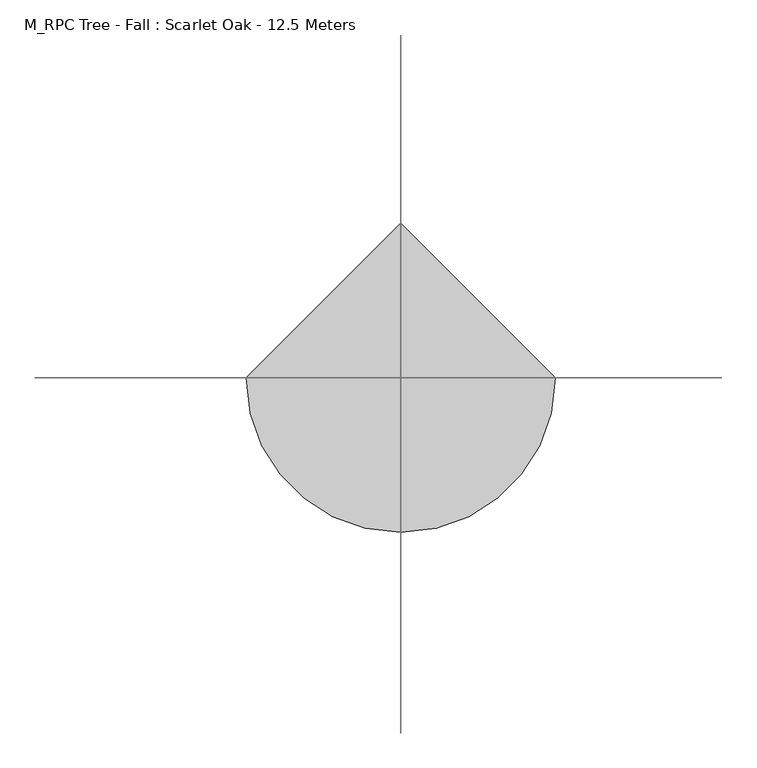
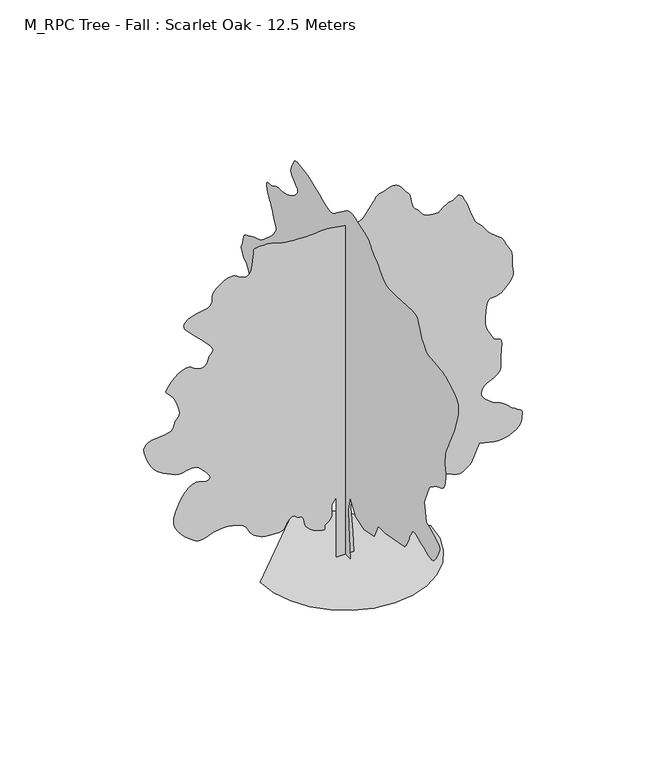
"""IFC4 building model written with IfcOpenShell, lengths in millimetres: geographic element geometry, M_RPC Tree - Fall : Scarlet Oak - 12.5 Meters."""

import ifcopenshell
import ifcopenshell.guid

model = None  # the IFC model being written
_history = None  # IfcOwnerHistory: only IFC2X3 demands one
_inside = {}  # id of a spatial element -> (the spatial element, [elements in it])
_under = {}  # id of a project, library or spatial element -> (it, [spatial elements below it])
_declared = {}  # id of a project -> (the project, [libraries it declares])
_typed = {}  # id of a type object -> (the type object, [elements of that type])
_made_of = {}  # id of a material, layer set ... -> (it, [elements and type objects made of it])


def new_model(schema):
    """Start an empty IFC model of exactly this schema.

    Asked for "IFC4X3", IfcOpenShell would pick the latest addendum, in which some entities
    have other attributes; the version numbers below select the first issue.
    IFC2X3 requires an IfcOwnerHistory on every rooted entity: one is made here for all.
    """
    global model, _history
    if schema == "IFC4X3":
        model = ifcopenshell.file(schema_version=(4, 3, 0, 0))
    else:
        model = ifcopenshell.file(schema=schema)
    _inside.clear()
    _under.clear()
    _declared.clear()
    _typed.clear()
    _made_of.clear()
    _history = None
    if model.schema == "IFC2X3":
        org = make("IfcOrganization", Name="unknown")
        user = make(
            "IfcPersonAndOrganization",
            ThePerson=make("IfcPerson", FamilyName="unknown"),
            TheOrganization=org,
        )
        app = make(
            "IfcApplication",
            ApplicationDeveloper=org,
            Version="unknown",
            ApplicationFullName="unknown",
            ApplicationIdentifier="unknown",
        )
        _history = make(
            "IfcOwnerHistory",
            OwningUser=user,
            OwningApplication=app,
            ChangeAction="ADDED",
            CreationDate=0,
        )
    return model


def make(cls, **values):
    """One entity of the class cls with the attributes given. An attribute that is None is left unset."""
    return model.create_entity(
        cls, **{name: value for name, value in values.items() if value is not None}
    )


def rooted(cls, **values):
    """An entity with a GlobalId (a new one), such as an element, a storey or a relation."""
    return make(cls, GlobalId=ifcopenshell.guid.new(), OwnerHistory=_history, **values)


def si_unit(unit_type, name, prefix=None):
    """IfcSIUnit, for example si_unit("LENGTHUNIT", "METRE", prefix="MILLI")."""
    return make("IfcSIUnit", UnitType=unit_type, Prefix=prefix, Name=name)


def assignment(units):
    """IfcUnitAssignment: the units of a project."""
    return None if units is None else make("IfcUnitAssignment", Units=units)


def point(xyz):
    """IfcCartesianPoint."""
    return None if xyz is None else make("IfcCartesianPoint", Coordinates=xyz)


def direction(xyz):
    """IfcDirection."""
    return None if xyz is None else make("IfcDirection", DirectionRatios=xyz)


def frame(location, z_axis=None, x_axis=None):
    """IfcAxis2Placement3D, a coordinate frame: its origin and axes. An axis left out is left unset."""
    return make(
        "IfcAxis2Placement3D",
        Location=point(location),
        Axis=direction(z_axis),
        RefDirection=direction(x_axis),
    )


def origin():
    """The frame at (0, 0, 0) with its axes left unset."""
    return frame((0.0, 0.0, 0.0))


def place(relative_to, where):
    """IfcLocalPlacement: puts the frame where relative to a parent placement (None: the world)."""
    return make(
        "IfcLocalPlacement", PlacementRelTo=relative_to, RelativePlacement=where
    )


def context(
    kind, dimensions, precision=None, world=None, true_north=None, identifier=None
):
    """IfcGeometricRepresentationContext, for example the 3D "Model" context."""
    return make(
        "IfcGeometricRepresentationContext",
        ContextIdentifier=identifier,
        ContextType=kind,
        CoordinateSpaceDimension=dimensions,
        Precision=precision,
        WorldCoordinateSystem=world,
        TrueNorth=true_north,
    )


def project(units=None, contexts=None):
    """IfcProject with its units and contexts."""
    return rooted(
        "IfcProject",
        Name="project",
        RepresentationContexts=contexts,
        UnitsInContext=assignment(units),
    )


def spatial(cls, under=None, at=None, **own):
    """A site, building, storey or space (cls), placed at a placement, below another one or the project."""
    s = rooted(cls, ObjectPlacement=at, **own)
    if under is not None:
        _under.setdefault(under.id(), (under, []))[1].append(s)
    return s


def point_list(points):
    """IfcCartesianPointList2D or 3D."""
    cls = (
        "IfcCartesianPointList2D" if len(points[0]) == 2 else "IfcCartesianPointList3D"
    )
    return make(cls, CoordList=points)


def triangles(points, corners, closed=None, point_numbers=None):
    """IfcTriangulatedFaceSet: each triangle names its three corners, points numbered from 1."""
    return make(
        "IfcTriangulatedFaceSet",
        Coordinates=point_list(points),
        Closed=closed,
        CoordIndex=corners,
        PnIndex=point_numbers,
    )


def shape(context_of_items, identifier, shape_type, items):
    """IfcShapeRepresentation: the items that make up one representation, for example the "Body"."""
    return make(
        "IfcShapeRepresentation",
        ContextOfItems=context_of_items,
        RepresentationIdentifier=identifier,
        RepresentationType=shape_type,
        Items=items,
    )


def source(mapping_origin, context_of_items, identifier, shape_type, items):
    """IfcRepresentationMap: a shape defined once, which mapped items show again and again."""
    return make(
        "IfcRepresentationMap",
        MappingOrigin=mapping_origin,
        MappedRepresentation=shape(context_of_items, identifier, shape_type, items),
    )


def transform(
    local_origin,
    x_axis=None,
    y_axis=None,
    z_axis=None,
    scale=None,
    scale2=None,
    scale3=None,
    uniform=True,
):
    """IfcCartesianTransformationOperator3D, or its non-uniform kind. x_axis, y_axis, z_axis: its Axis1, 2, 3."""
    if uniform:
        return make(
            "IfcCartesianTransformationOperator3D",
            Axis1=direction(x_axis),
            Axis2=direction(y_axis),
            LocalOrigin=point(local_origin),
            Scale=scale,
            Axis3=direction(z_axis),
        )
    return make(
        "IfcCartesianTransformationOperator3DnonUniform",
        Axis1=direction(x_axis),
        Axis2=direction(y_axis),
        LocalOrigin=point(local_origin),
        Scale=scale,
        Axis3=direction(z_axis),
        Scale2=scale2,
        Scale3=scale3,
    )


def mapped(mapping_source, mapping_target):
    """IfcMappedItem: shows the shape of a source again, moved by a transform."""
    return make(
        "IfcMappedItem", MappingSource=mapping_source, MappingTarget=mapping_target
    )


def made_of(thing, what):
    """Note that an element or type object is made of a material, layer set ...; save() writes the relation."""
    if what is not None:
        _made_of.setdefault(what.id(), (what, []))[1].append(thing)
    return thing


def element(
    cls,
    number,
    at=None,
    inside=None,
    cuts=None,
    type_object=None,
    material=None,
    context=None,
    identifier="Body",
    shape_type=None,
    held_by="IfcProductDefinitionShape",
    body=None,
    shapes=None,
    **own,
):
    """One element of the class cls, such as IfcWall. Its Tag is "e" and its number.

    at: its placement. inside: the storey or other place that contains it. cuts: it is an
    opening in that element (IfcRelVoidsElement). A single representation is given by context,
    identifier, shape_type and body (its items); several are given by shapes. held_by: the class
    of the entity that holds the representations. save() writes the other relations.
    """
    e = rooted(cls, Tag="e%d" % number, ObjectPlacement=at, **own)
    if body is not None:
        shapes = [shape(context, identifier, shape_type, body)]
    if shapes is not None:
        e.Representation = make(held_by, Representations=shapes)
    if inside is not None:
        _inside.setdefault(inside.id(), (inside, []))[1].append(e)
    if cuts is not None:
        rooted(
            "IfcRelVoidsElement", RelatingBuildingElement=cuts, RelatedOpeningElement=e
        )
    if type_object is not None:
        _typed.setdefault(type_object.id(), (type_object, []))[1].append(e)
    return made_of(e, material)


def aggregate(whole, parts):
    """IfcRelAggregates: a whole, such as a stair, and the parts it consists of."""
    return rooted("IfcRelAggregates", RelatingObject=whole, RelatedObjects=parts)


def save(model, path):
    """Write the relations noted so far, then the file.

    IfcRelAggregates (storeys below a building ...), IfcRelContainedInSpatialStructure (elements
    in a storey), IfcRelDefinesByType, IfcRelAssociatesMaterial and IfcRelDeclares: one each for
    every whole, place, type object, material and project.
    """
    for whole, parts in _under.values():
        aggregate(whole, parts)
    for where, things in _inside.values():
        rooted(
            "IfcRelContainedInSpatialStructure",
            RelatedElements=things,
            RelatingStructure=where,
        )
    for kind, things in _typed.values():
        rooted("IfcRelDefinesByType", RelatedObjects=things, RelatingType=kind)
    for what, things in _made_of.values():
        rooted("IfcRelAssociatesMaterial", RelatedObjects=things, RelatingMaterial=what)
    for by, libraries in _declared.values():
        rooted("IfcRelDeclares", RelatingContext=by, RelatedDefinitions=libraries)
    model.write(path)


def m_rpc_tree_fall_scarlet_oak_12_5_meters_13b38d7d(model_context):
    return source(origin(), model_context, "Body", "Tessellation", [
        triangles([(0.0172504, 306.0074844, 0.0), (0.0172504, -293.5650026, 0.0), (0.0172504, -196.8600042, 1141.1199549), (0.0172504, -177.5184886, 1682.6674953), (0.0172504, -293.5650026, 2185.5349113), (0.0172504, -603.0224945, 1682.6674953), (0.0172504, -1105.8875124, 1527.9400211), (0.0172504, -1686.1174301, 1663.3275421), (0.0172504, -1918.2099495, 2146.8525341), (0.0172504, -2324.3725124, 2146.8525341), (0.0172504, -3446.1498253, 2359.6049549), (0.0172504, -3487.4249222, 2409.394939), (0.0172504, -3527.7000801, 2459.5225479), (0.0172504, -3565.9250725, 2510.3249702), (0.0172504, -3601.0999603, 2562.1500046), (0.0172504, -3632.2248047, 2615.3249565), (0.0172504, -3658.2749588, 2670.2000954), (0.0172504, -3678.2499023, 2727.0748215), (0.0172504, -3697.649881, 2785.6750237), (0.0172504, -3722.1248405, 2845.2748741), (0.0172504, -3750.8248329, 2905.7249634), (0.0172504, -3782.89991, 2966.8500114), (0.0172504, -3817.5248314, 3028.475029), (0.0172504, -3853.8249413, 3090.4500252), (0.0172504, -3890.9999977, 3152.5750122), (0.0172504, -3908.7000801, 3172.6499496), (0.0172504, -3933.1750397, 3188.8498329), (0.0172504, -3971.1750458, 3197.2499016), (0.0172504, -4029.4749756, 3193.9748108), (0.0172504, -4114.8499969, 3175.1500877), (0.0172504, -4234.0499886, 3136.8498093), (0.0172504, -4393.8498276, 3075.2250824), (0.0172504, -4562.5749939, 3002.6998581), (0.0172504, -4706.2499451, 2937.9750298), (0.0172504, -4828.2750549, 2886.4249786), (0.0172504, -4932.0251175, 2853.4999535), (0.0172504, -5020.8999252, 2844.5999153), (0.0172504, -5098.249855, 2865.1248253), (0.0172504, -5167.4996979, 2920.4999336), (0.0172504, -5237.3750839, 3007.7248421), (0.0172504, -5309.5997452, 3113.9000473), (0.0172504, -5377.0996948, 3229.5499649), (0.0172504, -5432.7497864, 3345.1998825), (0.0172504, -5469.4498718, 3451.3750877), (0.0172504, -5480.1248016, 3538.6249947), (0.0172504, -5457.6250122, 3597.424894), (0.0172504, -5402.6498795, 3641.6998077), (0.0172504, -5323.3000717, 3691.0249947), (0.0172504, -5223.6747574, 3744.5999222), (0.0172504, -5107.774855, 3801.5499344), (0.0172504, -4979.7251129, 3861.0500816), (0.0172504, -4843.5499947, 3922.224836), (0.0172504, -4703.3248329, 3984.2498291), (0.0172504, -4587.2749397, 4641.8498062), (0.0172504, -4877.3749649, 5318.7747665), (0.0172504, -4886.5249878, 5331.7001404), (0.0172504, -4900.7247025, 5347.4747589), (0.0172504, -4925.0999588, 5369.0251877), (0.0172504, -4964.6748688, 5399.20009), (0.0172504, -5024.5497025, 5440.8498734), (0.0172504, -5109.8247299, 5496.8999405), (0.0172504, -5225.5246445, 5570.225116), (0.0172504, -5351.0501221, 5636.6501312), (0.0172504, -5462.3497238, 5680.0498077), (0.0172504, -5559.4501923, 5715.3499786), (0.0172504, -5642.3497833, 5757.424736), (0.0172504, -5711.0246613, 5821.1499161), (0.0172504, -5765.4998245, 5921.4001923), (0.0172504, -5805.7496933, 6073.0746552), (0.0172504, -5829.0500153, 6222.0498642), (0.0172504, -5835.7501877, 6317.5748474), (0.0172504, -5830.6249191, 6379.6001312), (0.0172504, -5818.3750854, 6428.1000778), (0.0172504, -5803.7748138, 6483.0246323), (0.0172504, -5791.5499786, 6564.3249023), (0.0172504, -5786.4247101, 6691.9996674), (0.0172504, -5788.2251816, 6832.849791), (0.0172504, -5796.1246994, 6949.6746368), (0.0172504, -5813.8247818, 7056.3751007), (0.0172504, -5845.0496201, 7166.7747574), (0.0172504, -5893.550148, 7294.7750839), (0.0172504, -5963.0249771, 7454.2496521), (0.0172504, -6057.1750443, 7659.049942), (0.0172504, -6146.5748199, 7844.1746887), (0.0172504, -6206.1746704, 7955.8748474), (0.0172504, -6246.4751175, 8024.9497009), (0.0172504, -6277.9999374, 8082.1746964), (0.0172504, -6311.2246536, 8158.3496979), (0.0172504, -6356.599791, 8284.2751511), (0.0172504, -6424.6747055, 8490.6997604), (0.0172504, -6498.0248795, 8729.4997192), (0.0172504, -6547.3747742, 8935.1499573), (0.0172504, -6565.2498459, 9112.3746048), (0.0172504, -6544.199968, 9265.925116), (0.0172504, -6476.8250107, 9400.5250397), (0.0172504, -6355.6498489, 9520.8996689), (0.0172504, -6173.2249374, 9631.8248749), (0.0172504, -5996.2246948, 9723.0001236), (0.0172504, -5879.7998245, 9785.7747803), (0.0172504, -5799.2250916, 9827.2001587), (0.0172504, -5729.799678, 9854.4496582), (0.0172504, -5646.85009, 9874.575174), (0.0172504, -5525.6749283, 9894.699527), (0.0172504, -5341.575119, 9921.9501892), (0.0172504, -5144.0999634, 9943.4244598), (0.0172504, -4990.9500092, 9951.725116), (0.0172504, -4869.5998581, 9962.0244873), (0.0172504, -4767.5499825, 9989.5995483), (0.0172504, -4672.2499855, 10049.6493713), (0.0172504, -4571.2000488, 10157.425351), (0.0172504, -4451.8750648, 10328.0998169), (0.0172504, -4347.6750298, 10515.7499908), (0.0172504, -4286.1000092, 10666.5500885), (0.0172504, -4245.8498497, 10783.8243256), (0.0172504, -4205.5749825, 10871.0003998), (0.0172504, -4143.9999619, 10931.4501984), (0.0172504, -4039.7999268, 10968.5502594), (0.0172504, -3871.650016, 10985.7003754), (0.0172504, -2943.2749969, 10927.6748474), (0.0172504, -2772.1499771, 10930.6746643), (0.0172504, -2632.8250511, 10930.2746887), (0.0172504, -2514.4500092, 10937.3242584), (0.0172504, -2406.244986, 10962.6250397), (0.0172504, -2297.3599171, 11017.0496246), (0.0172504, -2176.9724979, 11111.3752625), (0.0172504, -2034.2549011, 11256.4745453), (0.0172504, -1896.7275398, 11403.0249023), (0.0172504, -1793.7049038, 11502.8746216), (0.0172504, -1717.0749882, 11568.5752625), (0.0172504, -1658.7124168, 11612.6248993), (0.0172504, -1610.5024235, 11647.5250946), (0.0172504, -1564.3199226, 11685.7995026), (0.0172504, -1512.0500027, 11739.9996826), (0.0172504, -1461.8649845, 11803.9992645), (0.0172504, -1420.8125484, 11863.6002777), (0.0172504, -1379.087479, 11919.1503754), (0.0172504, -1326.8724976, 11970.9495392), (0.0172504, -1254.3574471, 12019.4000702), (0.0172504, -1151.7299904, 12064.7996246), (0.0172504, -1009.182514, 12107.4749268), (0.0172504, -849.1549999, 12154.4999634), (0.0172504, -699.9524792, 12206.6002716), (0.0172504, -560.5600064, 12254.6496643), (0.0172504, -429.9675053, 12289.4998627), (0.0172504, -307.1549798, 12302.0246796), (0.0172504, -191.1079934, 12283.0746735), (0.0172504, -80.8134993, 12223.5248199), (0.0172504, 499.4174812, 11798.0252106), (0.0172504, 562.2325061, 11740.8496307), (0.0172504, 623.0199657, 11688.7493225), (0.0172504, 689.217524, 11646.7751404), (0.0172504, 768.2749804, 11620.0500275), (0.0172504, 867.6299623, 11613.6248383), (0.0172504, 994.7275097, 11632.5748444), (0.0172504, 1157.0125168, 11681.9753174), (0.0172504, 1341.1749676, 11755.3243286), (0.0172504, 1526.6899521, 11837.8251068), (0.0172504, 1710.1749733, 11922.0246185), (0.0172504, 1888.2475342, 12000.4500641), (0.0172504, 2057.5249924, 12065.6995697), (0.0172504, 2214.6199093, 12110.3003357), (0.0172504, 2356.1550201, 12126.8249084), (0.0172504, 2484.8875694, 12135.849939), (0.0172504, 2604.4750374, 12156.3742676), (0.0172504, 2712.9248131, 12178.575238), (0.0172504, 2808.1498146, 12192.6743774), (0.0172504, 2888.1748718, 12188.8501923), (0.0172504, 2950.9248207, 12157.2753754), (0.0172504, 2994.400074, 12088.1249451), (0.0172504, 3033.2500282, 12001.2500153), (0.0172504, 3077.8499222, 11921.1246735), (0.0172504, 3119.7499809, 11845.0502472), (0.0172504, 3150.4998482, 11770.3245758), (0.0172504, 3161.6000427, 11694.2745667), (0.0172504, 3144.6249161, 11614.1503876), (0.0172504, 3091.124984, 11527.2498779), (0.0172504, 3009.2500397, 11447.6245056), (0.0172504, 2921.5998665, 11385.2492432), (0.0172504, 2841.4248184, 11331.3502075), (0.0172504, 2781.8749649, 11277.1000305), (0.0172504, 2756.1750801, 11213.7248291), (0.0172504, 2777.4749428, 11132.4251404), (0.0172504, 2859.0249069, 11024.3747589), (0.0172504, 2971.6250107, 10916.724353), (0.0172504, 3077.7999252, 10838.2000763), (0.0172504, 3178.2249001, 10782.3), (0.0172504, 3273.574894, 10742.6745117), (0.0172504, 3364.5248657, 10712.8251709), (0.0172504, 3451.7750633, 10686.4000397), (0.0172504, 3535.9498672, 10656.8995148), (0.0172504, 3620.024968, 10634.1753204), (0.0172504, 3706.4749237, 10626.6746155), (0.0172504, 3795.2750267, 10625.9502411), (0.0172504, 3886.4499847, 10623.5248077), (0.0172504, 3979.9997978, 10610.9499939), (0.0172504, 4075.9250473, 10579.7495728), (0.0172504, 4174.1998627, 10521.5252197), (0.0172504, 4275.775058, 10469.7993073), (0.0172504, 4375.6250679, 10451.2492767), (0.0172504, 4464.9998451, 10446.8995422), (0.0172504, 4535.0999268, 10437.8245148), (0.0172504, 4577.0999794, 10405.075351), (0.0172504, 4582.2249573, 10329.6753021), (0.0172504, 4541.6998146, 10192.7243591), (0.0172504, 4481.7999825, 10048.5994354), (0.0172504, 4432.0748199, 9951.4995483), (0.0172504, 4388.424868, 9882.1247131), (0.0172504, 4346.824791, 9821.224942), (0.0172504, 4303.174839, 9749.4996689), (0.0172504, 4253.4249687, 9647.6750702), (0.0172504, 4193.5498444, 9496.4499985), (0.0172504, 4130.2749275, 9347.6997757), (0.0172504, 4075.8250534, 9253.7496964), (0.0172504, 4034.1999779, 9195.999733), (0.0172504, 4009.500032, 9155.8498581), (0.0172504, 4005.7749687, 9114.7000443), (0.0172504, 4027.0998299, 9053.8996857), (0.0172504, 4077.4999512, 8954.8999146), (0.0172504, 4167.2249977, 8823.6747849), (0.0172504, 4293.1248711, 8684.3501495), (0.0172504, 4439.3499573, 8545.349913), (0.0172504, 4589.9500671, 8415.1497208), (0.0172504, 4729.0750053, 8302.1996384), (0.0172504, 4840.7748734, 8214.9747299), (0.0172504, 4909.1747681, 8161.9000626), (0.0172504, 4969.9001312, 8128.6997635), (0.0172504, 5061.0747986, 8095.1500671), (0.0172504, 5170.5250946, 8060.9248306), (0.0172504, 5286.0750183, 8025.6746567), (0.0172504, 5395.524733, 7989.0751465), (0.0172504, 5486.6999817, 7950.8001572), (0.0172504, 5547.4247635, 7910.4747116), (0.0172504, 5598.275148, 7876.9750122), (0.0172504, 5663.0246841, 7853.2997131), (0.0172504, 5734.1749924, 7830.2999542), (0.0172504, 5804.3247803, 7798.8251312), (0.0172504, 5866.0250839, 7749.7746368), (0.0172504, 5911.8001968, 7673.9746124), (0.0172504, 5934.2499893, 7562.325032), (0.0172504, 5952.6250305, 7450.1749008), (0.0172504, 5984.1998474, 7370.8500916), (0.0172504, 6018.4750809, 7312.1496048), (0.0172504, 6044.9996246, 7261.899765), (0.0172504, 6053.224704, 7207.9501511), (0.0172504, 6032.699794, 7138.074765), (0.0172504, 5972.9249542, 7040.1249298), (0.0172504, 5898.7248322, 6948.3747162), (0.0172504, 5838.7250061, 6893.5251572), (0.0172504, 5788.2001831, 6857.9500031), (0.0172504, 5742.4000717, 6824.0497467), (0.0172504, 5696.6249588, 6774.2498795), (0.0172504, 5646.1001358, 6690.9747299), (0.0172504, 5586.0997284, 6556.5997925), (0.0172504, 5520.6996506, 6421.9998688), (0.0172504, 5460.6998245, 6337.1498154), (0.0172504, 5411.5249191, 6283.0746277), (0.0172504, 5378.6001846, 6240.824881), (0.0172504, 5367.3247101, 6191.4999847), (0.0172504, 5383.09991, 6116.0999359), (0.0172504, 5431.3748703, 5995.7247253), (0.0172504, 5495.5000259, 5864.0496231), (0.0172504, 5555.8748291, 5761.8250488), (0.0172504, 5613.5747955, 5680.5747757), (0.0172504, 5669.5498672, 5611.8249023), (0.0172504, 5724.8749786, 5547.1497803), (0.0172504, 5780.5250702, 5478.0749268), (0.0172504, 5837.5250793, 5396.1496948), (0.0172504, 5903.6751114, 5315.3499756), (0.0172504, 5980.6500641, 5249.4249298), (0.0172504, 6060.324852, 5189.6000931), (0.0172504, 6134.5999695, 5127.0498413), (0.0172504, 6195.3247513, 5053.0247086), (0.0172504, 6234.3996918, 4958.6746536), (0.0172504, 6243.6997055, 4835.2499199), (0.0172504, 6251.5248093, 4738.3250221), (0.0172504, 6280.349794, 4706.349939), (0.0172504, 6313.2251129, 4704.825032), (0.0172504, 6333.2500534, 4699.249791), (0.0172504, 6323.4750687, 4655.0998695), (0.0172504, 6267.0500244, 4537.8750481), (0.0172504, 6146.999794, 4313.0498177), (0.0172504, 6021.4748978, 4060.8748032), (0.0172504, 5945.6998718, 3875.3750793), (0.0172504, 5898.3248566, 3742.6250427), (0.0172504, 5858.0749878, 3648.7999557), (0.0172504, 5803.5998245, 3580.0000854), (0.0172504, 5713.6000854, 3522.3748238), (0.0172504, 5566.7747452, 3462.0500175), (0.0172504, 5397.2496277, 3413.0998077), (0.0172504, 5248.0500137, 3392.5748978), (0.0172504, 5111.0246567, 3390.9999939), (0.0172504, 4978.0746323, 3398.8998024), (0.0172504, 4841.0498566, 3406.7749031), (0.0172504, 4691.8499519, 3405.1999992), (0.0172504, 4522.3498329, 3384.6750893), (0.0172504, 4353.2999771, 3366.3000481), (0.0172504, 4207.2498802, 3370.249807), (0.0172504, 4078.7998718, 3385.7000267), (0.0172504, 3962.5249924, 3401.8249146), (0.0172504, 3853.0249901, 3407.7998405), (0.0172504, 3744.8749054, 3392.799884), (0.0172504, 3632.6500694, 3345.9998337), (0.0172504, 3525.249939, 3296.2499634), (0.0172504, 3436.4248375, 3270.1998093), (0.0172504, 3368.249929, 3253.6249489), (0.0172504, 3322.75009, 3232.3250862), (0.0172504, 3301.9499062, 3192.0499283), (0.0172504, 3307.8748352, 3118.6500481), (0.0172504, 3342.5500443, 2997.8498634), (0.0172504, 3398.4748283, 2869.5248474), (0.0172504, 3465.5748024, 2778.7248665), (0.0172504, 3542.0000793, 2719.2500084), (0.0172504, 3625.8499031, 2684.8000763), (0.0172504, 3715.274968, 2669.1248703), (0.0172504, 3808.4248055, 2665.9500641), (0.0172504, 3903.4248207, 2669.0498749), (0.0172504, 4270.9250633, 2262.8999565), (0.0172504, 4299.7250496, 2217.1674282), (0.0172504, 4327.3498169, 2170.5925095), (0.0172504, 4352.6250183, 2122.3249615), (0.0172504, 4374.3248566, 2071.5174522), (0.0172504, 4391.2999832, 2017.3299168), (0.0172504, 4402.3498901, 1958.9124069), (0.0172504, 4406.2999397, 1895.4199162), (0.0172504, 4405.6249809, 1829.2200325), (0.0172504, 4400.8999786, 1763.6974331), (0.0172504, 4388.0248924, 1699.5299835), (0.0172504, 4362.9999664, 1637.3900265), (0.0172504, 4321.7248695, 1577.9574623), (0.0172504, 4260.1498489, 1521.9075405), (0.0172504, 4174.1998627, 1469.9175453), (0.0172504, 4092.2249245, 1425.7650078), (0.0172504, 4034.5999535, 1391.4249527), (0.0172504, 3985.4250481, 1364.8674168), (0.0172504, 3928.800016, 1344.0599659), (0.0172504, 3848.8499542, 1326.9749622), (0.0172504, 3729.6499626, 1311.5799717), (0.0172504, 3555.2998489, 1295.8475018), (0.0172504, 3356.9750359, 1298.1024513), (0.0172504, 3174.2248535, 1332.8375404), (0.0172504, 3003.6500908, 1392.27243), (0.0172504, 2841.8750816, 1468.6199501), (0.0172504, 2685.525032, 1554.1049938), (0.0172504, 2531.1748604, 1640.9424259), (0.0172504, 2375.4949734, 1721.3500179), (0.0172504, 2236.6674007, 1794.4849434), (0.0172504, 2129.3049133, 1863.5599422), (0.0172504, 2044.6099377, 1926.8850014), (0.0172504, 1973.7875164, 1982.7650208), (0.0172504, 1908.0399307, 2029.5099873), (0.0172504, 1838.5700432, 2065.4300331), (0.0172504, 1756.5824604, 2088.8299129), (0.0172504, 1666.4174698, 2108.5649002), (0.0172504, 1577.6074837, 2133.0375343), (0.0172504, 1489.134977, 2159.8799366), (0.0172504, 1399.9875114, 2186.7200134), (0.0172504, 1309.1449459, 2211.1925022), (0.0172504, 1215.5974583, 2230.9274895), (0.0172504, 1118.3299942, 2243.5575325), (0.0172504, 1018.8625191, 2250.1549496), (0.0172504, 919.3925005, 2253.7074944), (0.0172504, 819.9249527, 2254.7224033), (0.0172504, 720.4574776, 2253.7074944), (0.0172504, 620.9900024, 2251.1700039), (0.0172504, 521.5199839, 2247.6174591), (0.0172504, 422.0525087, 2243.5575325), (0.0172504, 228.6430025, 1953.4425373), (0.0172504, 189.960498, 1508.5999226), (280.4450004, 0.0006008, 0.0092122), (-299.78499, 0.0006008, 0.0092122), (-299.78499, 0.0004756, 2127.5199932), (-454.5149895, 0.0004756, 1914.7698978), (-454.5149895, 0.0005007, 1682.6775238), (-450.962481, 0.0005007, 1628.8274677), (-450.962481, 0.0005007, 1575.1449886), (-458.0674979, 0.0005007, 1521.8024597), (-475.8274967, 0.0005257, 1468.967458), (-507.8000001, 0.0005257, 1416.8100311), (-557.5350094, 0.0005257, 1365.4949947), (-628.5824896, 0.0005257, 1315.1974834), (-684.2375227, 0.0005257, 1262.982502), (-699.6325132, 0.0005257, 1210.0899456), (-696.0799685, 0.0005257, 1162.9524885), (-694.8950117, 0.0005257, 1127.990015), (-717.3950191, 0.0005257, 1111.6374521), (-784.8899546, 0.0005257, 1120.3224598), (-918.6974848, 0.0005257, 1160.4700092), (-1071.3399845, 0.0005257, 1223.0050003), (-1185.4124548, 0.0005257, 1293.6575191), (-1267.3424103, 0.0005257, 1371.0799736), (-1323.5625252, 0.0005257, 1453.9124176), (-1360.49748, 0.0005007, 1540.8049335), (-1384.5749348, 0.0005007, 1630.4049877), (-1402.2250202, 0.0005007, 1721.359901), (-1406.7349194, 0.0005007, 1746.1124599), (-1413.4449749, 0.0005007, 1770.1899147), (-1424.5524364, 0.0005007, 1792.9174519), (-1442.2599312, 0.0005007, 1813.6099388), (-1468.7599125, 0.0005007, 1831.5975037), (-1506.2599491, 0.0005007, 1846.2024261), (-1556.9524944, 0.0005007, 1856.747422), (-1607.6450397, 0.0005007, 1874.1124958), (-1647.509903, 0.0005007, 1903.3224861), (-1682.3024014, 0.0004756, 1934.8999191), (-1717.7700039, 0.0004756, 1959.3724079), (-1759.6674465, 0.0004756, 1967.2674202), (-1813.7424889, 0.0004756, 1949.1099529), (-1885.7500122, 0.0005007, 1895.4274738), (-1949.0724552, 0.0005007, 1820.3199944), (-1984.9925011, 0.0005007, 1746.902528), (-2011.0999191, 0.0005007, 1679.2374722), (-2044.9875309, 0.0005007, 1621.382428), (-2104.2525181, 0.0005007, 1577.402409), (-2206.4824699, 0.0005007, 1551.3499294), (-2369.2750042, 0.0005007, 1547.2900028), (-2549.149926, 0.0005007, 1559.2449417), (-2695.2000229, 0.0005007, 1578.979929), (-2813.8250496, 0.0005007, 1607.1750103), (-2911.4999016, 0.0005007, 1644.5025284), (-2994.6250603, 0.0005007, 1691.6425289), (-3069.5998444, 0.0005007, 1749.2724415), (-3142.9250198, 0.0005007, 1818.0648994), (-3205.1000038, 0.0005007, 1893.5100037), (-3249.7248962, 0.0004756, 1969.2975288), (-3287.549913, 0.0004756, 2043.389954), (-3329.4499718, 0.0004756, 2113.7624027), (-3386.2249947, 0.0004756, 2178.3824409), (-3468.7249008, 0.0004756, 2235.2224308), (-3587.7499031, 0.0004756, 2282.2499382), (-3707.4248657, 0.0004756, 2317.9974655), (-3794.2497986, 0.0004506, 2343.2600224), (-3862.8249733, 0.0004506, 2359.3875263), (-3927.674794, 0.0004506, 2367.7325111), (-4003.3248276, 0.0004506, 2369.6499813), (-4104.3750549, 0.0004506, 2366.4924706), (-4245.3498802, 0.0004506, 2359.6125126), (-4400.3500122, 0.0004506, 2335.1974331), (-4538.1250328, 0.0004756, 2289.8050003), (-4665.0498436, 0.0004756, 2240.3524956), (-4787.5749229, 0.0004756, 2203.7574909), (-4912.1501678, 0.0004756, 2196.9349422), (-5045.1501892, 0.0004756, 2236.7999508), (-5193.0498825, 0.0004506, 2340.272414), (-5347.7997391, 0.0004506, 2478.6475433), (-5490.6747391, 0.0004506, 2615.9999153), (-5612.2498764, 0.0004256, 2758.4499413), (-5703.0251495, 0.0004256, 2912.049868), (-5753.5499725, 0.0004256, 3082.8999046), (-5754.3499237, 0.0004005, 3277.0999695), (-5695.9250015, 0.0004005, 3500.7249825), (-5598.1501556, 0.0003755, 3726.2748779), (-5489.1998291, 0.0003755, 3919.6999901), (-5372.1499969, 0.0003505, 4077.2499664), (-5250.0248932, 0.0003505, 4195.2000343), (-5125.8499146, 0.0003505, 4269.8498383), (-5002.6998734, 0.0003505, 4297.4998947), (-4883.6001663, 0.0003505, 4274.3748528), (-4771.2750458, 0.0003505, 4235.4749016), (-4671.8250114, 0.0003505, 4218.8750427), (-4593.3248611, 0.0003505, 4225.6499199), (-4543.9249695, 0.0003505, 4256.7750549), (-4531.7498405, 0.0003505, 4313.2748039), (-4564.899852, 0.0003505, 4396.1749763), (-4651.4997986, 0.0003254, 4506.4749298), (-4752.500029, 0.0003254, 4617.0998634), (-4829.4749817, 0.0003254, 4702.3498924), (-4891.5496811, 0.0003254, 4765.2748306), (-4947.8747314, 0.0003254, 4808.9247826), (-5007.6001556, 0.0003254, 4836.3248543), (-5079.8248169, 0.0003004, 4850.5498581), (-5173.7248993, 0.0003004, 4854.5999016), (-5270.0248352, 0.0003254, 4845.5248741), (-5349.7751999, 0.0003254, 4824.5999886), (-5422.3998367, 0.0003254, 4801.3249557), (-5497.39991, 0.0003254, 4785.1247818), (-5584.2248428, 0.0003254, 4785.5250481), (-5692.3746368, 0.0003254, 4811.9748871), (-5831.3248764, 0.0003004, 4873.9498833), (-5978.7751785, 0.0003004, 4948.0997177), (-6108.6248108, 0.0003004, 5012.4248611), (-6224.624707, 0.0003004, 5078.4748993), (-6330.4496429, 0.0003004, 5157.6997147), (-6429.8749695, 0.0003004, 5261.5997681), (-6526.574881, 0.0002754, 5401.7249359), (-6624.2997299, 0.0002754, 5589.5750977), (-6705.1000305, 0.0002503, 5784.4998276), (-6749.6996338, 0.0002503, 5941.2001465), (-6759.8001801, 0.0002503, 6064.0746231), (-6737.074823, 0.0002253, 6157.4997345), (-6683.2246216, 0.0002253, 6225.8996292), (-6599.9500534, 0.0002253, 6273.6496216), (-6488.899855, 0.0002253, 6305.1750229), (-6357.7997177, 0.0002253, 6323.2750809), (-6219.2750336, 0.0002253, 6333.9500107), (-6082.3996674, 0.0002253, 6346.2748398), (-5956.3748016, 0.0002253, 6369.4501694), (-5850.3248795, 0.0002253, 6412.5998611), (-5773.3499268, 0.0002253, 6484.8251038), (-5734.5999664, 0.0002003, 6595.2997559), (-5705.9749695, 0.0002003, 6701.9746399), (-5661.749762, 0.0002003, 6771.4500504), (-5614.8497177, 0.0002003, 6825.699646), (-5578.0746368, 0.0002003, 6886.6999924), (-5564.3248947, 0.0001752, 6976.4747452), (-5586.4247086, 0.0001752, 7116.9998886), (-5657.2500366, 0.0001752, 7330.2496628), (-5757.5497284, 0.0001502, 7540.2996323), (-5853.4746872, 0.0001502, 7672.5247009), (-5935.8498917, 0.0001502, 7750.975145), (-5995.5747345, 0.0001252, 7799.6250824), (-6023.4747757, 0.0001252, 7842.5247894), (-6010.4499893, 0.0001252, 7903.7251236), (-5947.3497711, 0.0001252, 8007.1996216), (-5845.6501648, 0.0001252, 8136.3248795), (-5728.0247864, 0.0001001, 8253.9496765), (-5602.2749039, 0.0001001, 8353.3000076), (-5476.1750427, 0.0001001, 8427.6251221), (-5357.5497253, 0.0001001, 8470.1248535), (-5254.1246429, 0.0001001, 8474.0746124), (-5173.7248993, 0.0001001, 8432.6998123), (-5094.9000595, 0.0001001, 8371.00009), (-4997.8001724, 0.0001001, 8322.8501221), (-4892.5751999, 0.0001001, 8294.6500992), (-4789.3748131, 0.0001001, 8292.8496277), (-4698.3748444, 0.0001001, 8323.8750595), (-4629.6999664, 0.0001001, 8394.1248413), (-4593.4998505, 0.0001001, 8510.0497421), (-4560.3248405, 0.0001001, 8620.5749725), (-4508.224823, 7.51e-05, 8686.1000427), (-4458.4999512, 7.51e-05, 8730.2996704), (-4432.4497971, 7.51e-05, 8776.8747345), (-4451.3998032, 7.51e-05, 8849.4999527), (-4536.6498322, 7.51e-05, 8971.8750412), (-4709.5500343, 5.01e-05, 9167.6497192), (-4926.3498825, 5.01e-05, 9388.7995926), (-5120.1496811, 2.5e-05, 9575.0998489), (-5277.4249649, 2.5e-05, 9731.9745758), (-5384.5998184, 2.5e-05, 9864.8246063), (-5428.2000641, 0.0, 9979.0746094), (-5394.6497864, 0.0, 10080.1254181), (-5270.4248108, 0.0, 10173.3743774), (-5104.7500397, 0.0, 10245.2246429), (-4956.3497955, 0.0, 10286.2744629), (-4825.8749107, 0.0, 10308.3742767), (-4714.0000534, -2.5e-05, 10323.3745239), (-4621.3998917, -2.5e-05, 10343.1000641), (-4548.7749641, -2.5e-05, 10379.4245911), (-4496.7749405, -2.5e-05, 10444.1497101), (-4470.8500694, -2.5e-05, 10520.7252686), (-4466.9000198, -2.5e-05, 10587.8246613), (-4471.4000359, -2.5e-05, 10650.1999237), (-4470.8500694, -2.5e-05, 10712.5751862), (-4451.6747864, -5.01e-05, 10779.6745789), (-4400.3500122, -5.01e-05, 10856.2501373), (-4303.3748268, -5.01e-05, 10947.0248291), (-4184.6748047, -5.01e-05, 11036.8495789), (-4076.1250351, -5.01e-05, 11106.7243835), (-3976.0500389, -7.51e-05, 11155.5993073), (-3882.7249214, -7.51e-05, 11182.4999908), (-3794.4750755, -7.51e-05, 11186.3997528), (-3709.6000237, -7.51e-05, 11166.2498199), (-3626.4498665, -5.01e-05, 11121.1002502), (-3540.7248665, -5.01e-05, 11065.9001312), (-3452.3250298, -5.01e-05, 11022.8748505), (-3365.6000908, -5.01e-05, 11001.8249725), (-3284.9500717, -5.01e-05, 11012.5998962), (-3214.7999931, -5.01e-05, 11064.9746063), (-3159.5498772, -7.51e-05, 11168.7996643), (-3123.5750381, -7.51e-05, 11333.8500549), (-3102.0998955, -7.51e-05, 11511.0752838), (-3086.6999634, -0.0001001, 11648.0250641), (-3076.3750122, -0.0001001, 11749.4746857), (-3070.1248123, -0.0001001, 11820.1250244), (-3066.9000092, -0.0001001, 11864.7246277), (-3065.7250809, -0.0001001, 11888.0243683), (-3065.5500916, -0.0001001, 11894.7251221), (-3040.1248993, -0.0001001, 11898.674881), (-2971.0500458, -0.0001001, 11907.37435), (-2869.1498703, -0.0001001, 11916.0494019), (-2745.2748734, -0.0001001, 11920.0003235), (-2610.2249771, -0.0001001, 11914.4750793), (-2474.8323692, -0.0001001, 11894.7251221), (-2349.9349056, -0.0001001, 11856.0495758), (-2235.4099194, -0.0001001, 11813.024295), (-2120.5474537, -0.0001001, 11781.8494537), (-2000.2725277, -0.0001001, 11760.1251984), (-1869.507399, -0.0001001, 11745.5249268), (-1723.1824642, -0.0001001, 11735.6743652), (-1556.2175102, -0.0001001, 11728.174823), (-1363.5400269, -0.0001001, 11720.6752808), (-1177.5749971, -0.0001001, 11719.599765), (-1024.4249702, -0.0001001, 11728.6747925), (-889.5449764, -0.0001001, 11741.475174), (-758.3875025, -0.0001001, 11751.5745575), (-616.4049625, -0.0001001, 11752.5244995), (-449.0450109, -0.0001001, 11737.9253906), (-241.7632409, -0.0001001, 11701.3252991), (-32.2257492, -0.0001001, 11657.8000488), (136.7124946, -0.0001001, 11627.7995544), (271.8174929, -0.0001001, 11613.0248749), (379.8574825, -0.0001001, 11615.1503265), (467.5974758, -0.0001001, 11635.9246399), (541.8025031, -0.0001001, 11676.9744598), (609.2425, -0.0001001, 11739.9996826), (899.3574589, -0.0001252, 12107.4749268), (942.8899761, -0.0001252, 12164.1493744), (977.6249926, -0.0001252, 12217.4496094), (1008.9749685, -0.0001252, 12266.3245331), (1042.3574512, -0.0001252, 12309.7997864), (1083.1825029, -0.0001252, 12346.8498505), (1136.864982, -0.0001252, 12376.4503693), (1208.8149508, -0.0001252, 12397.6002411), (1297.0049892, -0.0001502, 12421.8499237), (1393.3149536, -0.0001502, 12454.2246918), (1494.0224693, -0.0001502, 12483.8752075), (1595.4100307, -0.0001502, 12499.9998047), (1693.7499584, -0.0001502, 12491.7747253), (1785.3224213, -0.0001502, 12448.349469), (1866.4099136, -0.0001252, 12358.9246948), (1938.4149662, -0.0001252, 12256.9251068), (2004.3324543, -0.0001252, 12177.5752991), (2062.8075188, -0.0001252, 12112.7746033), (2112.4850098, -0.0001252, 12054.4246765), (2152.0125389, -0.0001252, 11994.3748535), (2180.0374271, -0.0001001, 11924.5000488), (2195.2049606, -0.0001001, 11836.6995941), (2205.7499565, -0.0001001, 11745.6993347), (2220.3550243, -0.0001001, 11669.9248901), (2238.3424438, -0.0001001, 11606.8252533), (2259.0349308, -7.51e-05, 11553.8749969), (2281.7599972, -7.51e-05, 11508.5242767), (2305.8374519, -7.51e-05, 11468.274408), (2330.5924816, -7.51e-05, 11430.5499664), (2355.6274361, -7.51e-05, 11413.5742584), (2381.6799156, -7.51e-05, 11394.2242767), (2409.760033, -7.51e-05, 11370.1501648), (2440.8873482, -7.51e-05, 11338.9753235), (2476.0724098, -7.51e-05, 11298.3243164), (2516.3248947, -7.51e-05, 11245.8251953), (2562.6749725, -7.51e-05, 11179.1246155), (2631.3748489, -5.01e-05, 11115.7249969), (2728.4750267, -5.01e-05, 11072.3253204), (2839.7749191, -5.01e-05, 11045.1246552), (2951.0748116, -5.01e-05, 11030.4743866), (3048.1749893, -5.01e-05, 11024.6003265), (3116.8748657, -5.01e-05, 11023.8247925), (3142.9250198, -5.01e-05, 11024.4003387), (3156.2750771, -5.01e-05, 11038.3250702), (3192.9998703, -5.01e-05, 11074.2252045), (3247.9750031, -5.01e-05, 11123.3501129), (3316.1499115, -7.51e-05, 11176.8503357), (3392.4249069, -7.51e-05, 11225.9752441), (3471.7750053, -7.51e-05, 11261.8997955), (3549.0749382, -7.51e-05, 11275.824527), (3618.3750687, -7.51e-05, 11292.800235), (3679.549823, -7.51e-05, 11331.0746429), (3736.3498444, -7.51e-05, 11371.7244873), (3792.4499084, -7.51e-05, 11395.8253418), (3851.6000771, -7.51e-05, 11384.3748779), (3917.5248322, -7.51e-05, 11318.4498322), (3993.9248199, -7.51e-05, 11179.1246155), (4065.8750793, -5.01e-05, 11015.4253052), (4119.5500008, -5.01e-05, 10883.1996552), (4160.3748344, -5.01e-05, 10773.6249481), (4193.7498322, -2.5e-05, 10677.9493927), (4225.0999535, -2.5e-05, 10587.3246918), (4259.8498672, -2.5e-05, 10493.0002167), (4303.3748268, -2.5e-05, 10386.1253448), (4348.1000038, 0.0, 10292.3496735), (4386.3749931, 0.0, 10232.749823), (4423.6500435, 0.0, 10191.7744171), (4465.3248253, 0.0, 10153.824408), (4516.799881, 0.0, 10103.3495819), (4583.4998795, 0.0, 10024.7997253), (4670.850071, 0.0, 9902.6002075), (4778.3749031, 2.5e-05, 9766.6003693), (4896.3999664, 2.5e-05, 9652.9247498), (5016.4501968, 2.5e-05, 9555.474884), (5130.0746567, 5.01e-05, 9468.1999786), (5228.8000259, 5.01e-05, 9384.974826), (5304.2000748, 5.01e-05, 9299.6997986), (5347.7997391, 5.01e-05, 9206.3246841), (5382.0249756, 5.01e-05, 9114.7500412), (5429.774968, 7.51e-05, 9032.6498199), (5483.3001892, 7.51e-05, 8950.5495987), (5534.7749542, 7.51e-05, 8858.9749557), (5576.449736, 7.51e-05, 8748.4747238), (5600.5250107, 0.0001001, 8609.5250656), (5599.22509, 0.0001001, 8432.6998123), (5596.5746704, 0.0001001, 8262.7497208), (5611.174942, 0.0001252, 8138.7997284), (5627.1251312, 0.0001252, 8042.949765), (5628.5500443, 0.0001252, 7957.224765), (5599.5000732, 0.0001252, 7863.7496567), (5524.1250229, 0.0001502, 7744.5249573), (5386.474704, 0.0001502, 7581.6750137), (5223.124791, 0.0001502, 7444.9496384), (5081.4247192, 0.0001502, 7390.0750809), (4961.7000504, 0.0001502, 7378.1746445), (4864.3248894, 0.0001502, 7370.3501221), (4789.5997993, 0.0001752, 7327.6498215), (4737.9000481, 0.0001752, 7211.2249512), (4709.5250359, 0.0001752, 6982.1249817), (4698.9248108, 0.0002003, 6728.5997589), (4700.5250038, 0.0002003, 6550.1751846), (4714.6000168, 0.0002253, 6424.8996918), (4741.5748238, 0.0002253, 6330.7246262), (4781.7249893, 0.0002253, 6245.7001648), (4835.3999107, 0.0002253, 6147.7997452), (4902.950148, 0.0002503, 6015.074707), (4980.0250946, 0.0002503, 5899.6497757), (5057.7999985, 0.0002503, 5847.1500732), (5129.7996735, 0.0002503, 5825.7746338), (5189.6250916, 0.0002503, 5803.7248169), (5230.8499008, 0.0002503, 5749.1996567), (5247.0250763, 0.0002754, 5630.3749329), (5231.7498459, 0.0002754, 5415.4996765), (5210.9999496, 0.0003004, 5178.6001831), (5207.8251434, 0.0003004, 5005.3247131), (5211.4499222, 0.0003004, 4881.0997375), (5210.9999496, 0.0003254, 4791.3999802), (5195.6497238, 0.0003254, 4721.6498772), (5154.5999039, 0.0003254, 4657.3000259), (5077.0249878, 0.0003254, 4583.8248596), (4983.2998947, 0.0003254, 4514.9249954), (4900.3997223, 0.0003254, 4468.3499313), (4827.3248222, 0.0003254, 4435.6498924), (4763.0499664, 0.0003505, 4408.3498146), (4706.5499268, 0.0003505, 4378.0249214), (4656.8250549, 0.0003505, 4336.1748596), (4612.8248337, 0.0003505, 4274.3748528), (4577.8749321, 0.0003505, 4202.8248596), (4558.1249748, 0.0003505, 4135.32491), (4557.0000435, 0.0003505, 4068.8498978), (4577.8749321, 0.0003755, 4000.3250107), (4624.1000175, 0.0003755, 3926.7498505), (4699.0998001, 0.0003755, 3845.024897), (4806.2499458, 0.0003755, 3752.1750412), (4919.7997009, 0.0003755, 3670.8000664), (5016.1246353, 0.0003755, 3617.4998314), (5101.5996506, 0.0004005, 3580.1250778), (5182.6999329, 0.0004005, 3546.4748062), (5265.8000931, 0.0004005, 3504.3500519), (5357.374736, 0.0004005, 3441.5748138), (5463.8246338, 0.0004005, 3345.9998337), (5576.8497116, 0.0004005, 3247.2750458), (5681.0497467, 0.0004005, 3176.6249977), (5772.3999847, 0.0004256, 3124.2249985), (5846.8250931, 0.0004256, 3080.3000633), (5900.2747375, 0.0004256, 3035.0249199), (5928.6997467, 0.0004256, 2978.5748772), (5928.0247879, 0.0004256, 2901.1499519), (5916.924884, 0.0004256, 2813.2500847), (5910.1997131, 0.0004506, 2730.7498878), (5898.0748718, 0.0004506, 2651.975045), (5870.7247971, 0.0004506, 2575.2500771), (5818.350087, 0.0004506, 2498.8349739), (5731.1251785, 0.0004506, 2421.0748947), (5599.22509, 0.0004506, 2340.272414), (5441.7248199, 0.0004756, 2274.8624531), (5284.2501297, 0.0004756, 2240.917432), (5126.7498596, 0.0004756, 2233.1924675), (4969.2501709, 0.0004756, 2246.4425308), (4811.7748993, 0.0004756, 2275.4249187), (4654.2749199, 0.0004756, 2314.8975094), (4496.7749405, 0.0004506, 2359.6125126), (4225.9998985, 0.0005007, 1760.0424236), (4159.6498787, 0.0005007, 1702.5250042), (4092.9248817, 0.0005007, 1648.0549278), (4025.5499245, 0.0005007, 1599.675032), (3957.1500298, 0.0005007, 1560.4274277), (3887.3999268, 0.0005007, 1533.3625099), (3815.9499275, 0.0005007, 1521.5225349), (3742.4750519, 0.0005007, 1527.9499043), (3682.5999275, 0.0005007, 1542.5525013), (3644.6999153, 0.0005007, 1554.7899811), (3617.6498222, 0.0005007, 1567.0274609), (3590.2500412, 0.0005007, 1581.6299126), (3551.3248009, 0.0005007, 1600.9724819), (3489.750071, 0.0005007, 1627.4175247), (3394.3500801, 0.0005007, 1663.3374252), (3270.0748169, 0.0005007, 1715.4949974), (3134.2999649, 0.0005007, 1784.5699963), (2994.450071, 0.0005007, 1863.794957), (2857.9999695, 0.0004756, 1946.4024147), (2732.3500809, 0.0004756, 2025.6275208), (2624.9999474, 0.0004756, 2094.7025196), (2543.3499893, 0.0004756, 2146.8624172), (2474.2123489, 0.0004756, 2192.817461), (2400.0074306, 0.0004756, 2246.8925034), (2321.5699219, 0.0004756, 2307.7374813), (2239.7525322, 0.0004506, 2373.9924488), (2155.3950359, 0.0004506, 2444.3074883), (2069.3475266, 0.0004506, 2517.3248337), (1982.4550106, 0.0004506, 2591.6999451), (1963.1124413, 0.0004256, 2881.8249687), (1576.2924477, 0.0004256, 2920.4999336), (880.0149622, 0.0004256, 2862.474987), (415.8325032, 0.0004506, 2611.0499268), (222.421489, 0.0004756, 2146.8624172), (183.7397477, 0.0005007, 1605.3124786), (241.7622416, 0.0005507, 715.6274672), (-2855.9000977, 0.0, 0.0224297), (-2780.4000549, -654.3849844, 0.0224297), (-2565.3750984, -1255.3350037, 0.0224297), (-2228.0499035, -1785.6274899, 0.0224297), (-1785.6274899, -2228.0499035, 0.0224297), (-1255.3350037, -2565.3750984, 0.0224297), (-654.3849844, -2780.4000549, 0.0224297), (0.0001248, -2855.9000977, 0.0224297), (654.3849844, -2780.4000549, 0.0224297), (1255.3350037, -2565.3750984, 0.0224297), (1785.6274899, -2228.0499035, 0.0224297), (2228.0499035, -1785.6274899, 0.0224297), (2565.3750984, -1255.3350037, 0.0224297), (2780.4000549, -654.3849844, 0.0224297), (2855.9000977, 0.0002503, 0.0224297), (-0.0003745, 2855.9000977, 0.0224297)], [[1, 2, 3], [368, 1, 3], [368, 3, 4], [367, 368, 4], [367, 4, 5], [277, 278, 279], [366, 367, 5], [276, 277, 279], [276, 279, 280], [7, 8, 9], [6, 7, 9], [5, 6, 9], [315, 316, 317], [201, 202, 203], [200, 201, 203], [200, 203, 204], [199, 200, 204], [199, 204, 205], [198, 199, 205], [198, 205, 206], [198, 206, 207], [197, 198, 207], [197, 207, 208], [275, 276, 280], [196, 197, 208], [195, 196, 208], [194, 195, 208], [194, 208, 209], [193, 194, 209], [192, 193, 209], [192, 209, 210], [191, 192, 210], [191, 210, 211], [191, 211, 212], [190, 191, 212], [190, 212, 213], [190, 213, 214], [189, 190, 214], [189, 214, 215], [188, 189, 215], [187, 188, 215], [186, 187, 215], [10, 11, 12], [314, 315, 317], [10, 12, 13], [10, 13, 14], [10, 14, 15], [10, 15, 16], [10, 16, 17], [10, 17, 18], [10, 18, 19], [10, 19, 20], [10, 20, 21], [10, 21, 22], [185, 186, 215], [185, 215, 216], [275, 280, 281], [10, 22, 23], [167, 168, 169], [166, 167, 169], [165, 166, 169], [165, 169, 170], [164, 165, 170], [164, 170, 171], [163, 164, 171], [163, 171, 172], [163, 172, 173], [163, 173, 174], [163, 174, 175], [163, 175, 176], [163, 176, 177], [163, 177, 178], [163, 178, 179], [163, 179, 180], [162, 163, 180], [161, 162, 180], [160, 161, 180], [159, 160, 180], [159, 180, 181], [158, 159, 181], [157, 158, 181], [156, 157, 181], [156, 181, 182], [155, 156, 182], [154, 155, 182], [154, 182, 183], [9, 10, 23], [9, 23, 24], [9, 24, 25], [45, 46, 47], [44, 45, 47], [44, 47, 48], [43, 44, 48], [43, 48, 49], [42, 43, 49], [42, 49, 50], [41, 42, 50], [40, 41, 50], [40, 50, 51], [39, 40, 51], [38, 39, 51], [37, 38, 51], [36, 37, 51], [35, 36, 51], [34, 35, 51], [33, 34, 51], [33, 51, 52], [32, 33, 52], [32, 52, 53], [31, 32, 53], [30, 31, 53], [29, 30, 53], [28, 29, 53], [28, 53, 54], [27, 28, 54], [26, 27, 54], [5, 9, 25], [5, 25, 26], [5, 26, 54], [5, 54, 55], [366, 5, 55], [365, 366, 55], [364, 365, 55], [363, 364, 55], [362, 363, 55], [361, 362, 55], [361, 55, 56], [153, 154, 183], [153, 183, 184], [313, 314, 317], [360, 361, 56], [184, 185, 216], [153, 184, 216], [152, 153, 216], [152, 216, 217], [243, 244, 245], [242, 243, 245], [242, 245, 246], [241, 242, 246], [241, 246, 247], [241, 247, 248], [240, 241, 248], [240, 248, 249], [240, 249, 250], [239, 240, 250], [239, 250, 251], [238, 239, 251], [237, 238, 251], [236, 237, 251], [235, 236, 251], [234, 235, 251], [233, 234, 251], [232, 233, 251], [231, 232, 251], [230, 231, 251], [229, 230, 251], [228, 229, 251], [228, 251, 252], [227, 228, 252], [226, 227, 252], [226, 252, 253], [226, 253, 254], [226, 254, 255], [226, 255, 256], [226, 256, 257], [225, 226, 257], [224, 225, 257], [223, 224, 257], [222, 223, 257], [222, 257, 258], [221, 222, 258], [220, 221, 258], [115, 116, 117], [114, 115, 117], [114, 117, 118], [113, 114, 118], [113, 118, 119], [112, 113, 119], [111, 112, 119], [110, 111, 119], [152, 217, 218], [313, 317, 318], [313, 318, 319], [313, 319, 320], [313, 320, 321], [313, 321, 322], [313, 322, 323], [313, 323, 324], [313, 324, 325], [313, 325, 326], [313, 326, 327], [313, 327, 328], [313, 328, 329], [313, 329, 330], [313, 330, 331], [313, 331, 332], [313, 332, 333], [313, 333, 334], [313, 334, 335], [313, 335, 336], [313, 336, 337], [313, 337, 338], [313, 338, 339], [313, 339, 340], [313, 340, 341], [312, 313, 341], [312, 341, 342], [312, 342, 343], [311, 312, 343], [311, 343, 344], [311, 344, 345], [310, 311, 345], [310, 345, 346], [310, 346, 347], [310, 347, 348], [309, 310, 348], [309, 348, 349], [309, 349, 350], [308, 309, 350], [308, 350, 351], [307, 308, 351], [307, 351, 352], [307, 352, 353], [307, 353, 354], [307, 354, 355], [307, 355, 356], [307, 356, 357], [307, 357, 358], [306, 307, 358], [306, 358, 359], [306, 359, 360], [306, 360, 56], [305, 306, 56], [305, 56, 57], [304, 305, 57], [303, 304, 57], [302, 303, 57], [301, 302, 57], [301, 57, 58], [301, 58, 59], [110, 119, 120], [109, 110, 120], [109, 120, 121], [301, 59, 60], [300, 301, 60], [300, 60, 61], [151, 152, 218], [109, 121, 122], [300, 61, 62], [145, 146, 147], [144, 145, 147], [143, 144, 147], [143, 147, 148], [142, 143, 148], [141, 142, 148], [140, 141, 148], [140, 148, 149], [139, 140, 149], [138, 139, 149], [137, 138, 149], [136, 137, 149], [135, 136, 149], [134, 135, 149], [133, 134, 149], [132, 133, 149], [132, 149, 150], [131, 132, 150], [130, 131, 150], [129, 130, 150], [128, 129, 150], [127, 128, 150], [126, 127, 150], [126, 150, 151], [126, 151, 218], [125, 126, 218], [124, 125, 218], [123, 124, 218], [123, 218, 219], [122, 123, 219], [109, 122, 219], [108, 109, 219], [108, 219, 220], [108, 220, 258], [108, 258, 259], [108, 259, 260], [108, 260, 261], [108, 261, 262], [107, 108, 262], [107, 262, 263], [107, 263, 264], [106, 107, 264], [106, 264, 265], [106, 265, 266], [106, 266, 267], [106, 267, 268], [105, 106, 268], [104, 105, 268], [103, 104, 268], [102, 103, 268], [101, 102, 268], [100, 101, 268], [99, 100, 268], [98, 99, 268], [97, 98, 268], [96, 97, 268], [95, 96, 268], [94, 95, 268], [93, 94, 268], [92, 93, 268], [91, 92, 268], [90, 91, 268], [89, 90, 268], [88, 89, 268], [87, 88, 268], [86, 87, 268], [85, 86, 268], [84, 85, 268], [83, 84, 268], [82, 83, 268], [81, 82, 268], [80, 81, 268], [79, 80, 268], [78, 79, 268], [77, 78, 268], [76, 77, 268], [75, 76, 268], [74, 75, 268], [73, 74, 268], [72, 73, 268], [71, 72, 268], [70, 71, 268], [69, 70, 268], [68, 69, 268], [67, 68, 268], [66, 67, 268], [65, 66, 268], [64, 65, 268], [63, 64, 268], [62, 63, 268], [300, 62, 268], [299, 300, 268], [298, 299, 268], [297, 298, 268], [296, 297, 268], [295, 296, 268], [294, 295, 268], [293, 294, 268], [292, 293, 268], [291, 292, 268], [290, 291, 268], [289, 290, 268], [288, 289, 268], [287, 288, 268], [286, 287, 268], [285, 286, 268], [284, 285, 268], [283, 284, 268], [282, 283, 268], [281, 282, 268], [275, 281, 268], [275, 268, 269], [274, 275, 269], [274, 269, 270], [274, 270, 271], [273, 274, 271], [272, 273, 271], [802, 369, 370], [802, 370, 371], [801, 802, 371], [800, 801, 371], [575, 576, 577], [799, 800, 371], [574, 575, 577], [383, 384, 385], [383, 385, 386], [382, 383, 386], [382, 386, 387], [381, 382, 387], [381, 387, 388], [794, 795, 796], [510, 511, 512], [574, 577, 578], [573, 574, 578], [572, 573, 578], [572, 578, 579], [571, 572, 579], [571, 579, 580], [570, 571, 580], [570, 580, 581], [570, 581, 582], [569, 570, 582], [569, 582, 583], [569, 583, 584], [568, 569, 584], [568, 584, 585], [509, 510, 512], [509, 512, 513], [508, 509, 513], [508, 513, 514], [508, 514, 515], [507, 508, 515], [507, 515, 516], [507, 516, 517], [507, 517, 518], [507, 518, 519], [507, 519, 520], [507, 520, 521], [507, 521, 522], [506, 507, 522], [506, 522, 523], [505, 506, 523], [505, 523, 524], [504, 505, 524], [568, 585, 586], [504, 524, 525], [538, 539, 540], [538, 540, 541], [537, 538, 541], [537, 541, 542], [536, 537, 542], [536, 542, 543], [536, 543, 544], [535, 536, 544], [535, 544, 545], [535, 545, 546], [534, 535, 546], [534, 546, 547], [533, 534, 547], [533, 547, 548], [381, 388, 389], [380, 381, 389], [380, 389, 390], [380, 390, 391], [380, 391, 392], [380, 392, 393], [379, 380, 393], [378, 379, 393], [377, 378, 393], [376, 377, 393], [375, 376, 393], [374, 375, 393], [373, 374, 393], [372, 373, 393], [372, 393, 394], [372, 394, 395], [372, 395, 396], [372, 396, 397], [372, 397, 398], [371, 372, 398], [371, 398, 399], [532, 533, 548], [371, 399, 400], [567, 568, 586], [567, 586, 587], [657, 658, 659], [657, 659, 660], [656, 657, 660], [656, 660, 661], [655, 656, 661], [655, 661, 662], [654, 655, 662], [654, 662, 663], [653, 654, 663], [652, 653, 663], [651, 652, 663], [650, 651, 663], [649, 650, 663], [649, 663, 664], [648, 649, 664], [647, 648, 664], [647, 664, 665], [647, 665, 666], [647, 666, 667], [647, 667, 668], [647, 668, 669], [793, 794, 796], [713, 714, 715], [713, 715, 716], [712, 713, 716], [712, 716, 717], [711, 712, 717], [646, 647, 669], [711, 717, 718], [567, 587, 588], [645, 646, 669], [645, 669, 670], [750, 751, 752], [749, 750, 752], [748, 749, 752], [748, 752, 753], [747, 748, 753], [747, 753, 754], [747, 754, 755], [747, 755, 756], [747, 756, 757], [747, 757, 758], [747, 758, 759], [747, 759, 760], [746, 747, 760], [746, 760, 761], [746, 761, 762], [745, 746, 762], [745, 762, 763], [745, 763, 764], [744, 745, 764], [743, 744, 764], [743, 764, 765], [742, 743, 765], [741, 742, 765], [741, 765, 766], [740, 741, 766], [739, 740, 766], [738, 739, 766], [737, 738, 766], [736, 737, 766], [735, 736, 766], [644, 645, 670], [567, 588, 589], [792, 793, 796], [371, 400, 401], [371, 401, 402], [371, 402, 403], [371, 403, 404], [371, 404, 405], [799, 371, 405], [799, 405, 406], [766, 767, 768], [488, 489, 490], [488, 490, 491], [487, 488, 491], [487, 491, 492], [486, 487, 492], [486, 492, 493], [485, 486, 493], [485, 493, 494], [485, 494, 495], [484, 485, 495], [483, 484, 495], [483, 495, 496], [482, 483, 496], [481, 482, 496], [480, 481, 496], [479, 480, 496], [479, 496, 497], [478, 479, 497], [477, 478, 497], [476, 477, 497], [475, 476, 497], [474, 475, 497], [473, 474, 497], [472, 473, 497], [471, 472, 497], [471, 497, 498], [470, 471, 498], [469, 470, 498], [469, 498, 499], [468, 469, 499], [468, 499, 500], [468, 500, 501], [468, 501, 502], [468, 502, 503], [467, 468, 503], [466, 467, 503], [466, 503, 504], [466, 504, 525], [465, 466, 525], [465, 525, 526], [464, 465, 526], [463, 464, 526], [735, 766, 768], [735, 768, 769], [735, 769, 770], [735, 770, 771], [735, 771, 772], [735, 772, 773], [735, 773, 774], [735, 774, 775], [735, 775, 776], [735, 776, 777], [735, 777, 778], [735, 778, 779], [735, 779, 780], [735, 780, 781], [735, 781, 782], [735, 782, 783], [735, 783, 784], [735, 784, 785], [735, 785, 786], [735, 786, 787], [735, 787, 788], [735, 788, 789], [735, 789, 790], [735, 790, 791], [735, 791, 792], [735, 792, 796], [734, 735, 796], [733, 734, 796], [732, 733, 796], [731, 732, 796], [731, 796, 797], [730, 731, 797], [567, 589, 590], [455, 456, 457], [454, 455, 457], [453, 454, 457], [453, 457, 458], [452, 453, 458], [451, 452, 458], [451, 458, 459], [450, 451, 459], [449, 450, 459], [448, 449, 459], [447, 448, 459], [446, 447, 459], [445, 446, 459], [444, 445, 459], [443, 444, 459], [442, 443, 459], [441, 442, 459], [440, 441, 459], [439, 440, 459], [438, 439, 459], [437, 438, 459], [437, 459, 460], [436, 437, 460], [435, 436, 460], [434, 435, 460], [434, 460, 461], [433, 434, 461], [432, 433, 461], [431, 432, 461], [430, 431, 461], [429, 430, 461], [428, 429, 461], [428, 461, 462], [427, 428, 462], [411, 412, 413], [411, 413, 414], [410, 411, 414], [410, 414, 415], [409, 410, 415], [409, 415, 416], [409, 416, 417], [408, 409, 417], [408, 417, 418], [408, 418, 419], [408, 419, 420], [408, 420, 421], [408, 421, 422], [408, 422, 423], [408, 423, 424], [408, 424, 425], [408, 425, 426], [407, 408, 426], [407, 426, 427], [407, 427, 462], [406, 407, 462], [799, 406, 462], [799, 462, 463], [799, 463, 526], [798, 799, 526], [798, 526, 527], [798, 527, 528], [798, 528, 529], [798, 529, 530], [798, 530, 531], [797, 798, 531], [730, 797, 531], [729, 730, 531], [728, 729, 531], [728, 531, 532], [728, 532, 548], [728, 548, 549], [728, 549, 550], [727, 728, 550], [726, 727, 550], [725, 726, 550], [724, 725, 550], [723, 724, 550], [722, 723, 550], [721, 722, 550], [720, 721, 550], [719, 720, 550], [718, 719, 550], [711, 718, 550], [710, 711, 550], [709, 710, 550], [708, 709, 550], [707, 708, 550], [706, 707, 550], [705, 706, 550], [704, 705, 550], [703, 704, 550], [702, 703, 550], [701, 702, 550], [701, 550, 551], [701, 551, 552], [701, 552, 553], [701, 553, 554], [701, 554, 555], [701, 555, 556], [701, 556, 557], [701, 557, 558], [701, 558, 559], [700, 701, 559], [699, 700, 559], [698, 699, 559], [697, 698, 559], [696, 697, 559], [617, 618, 619], [616, 617, 619], [615, 616, 619], [615, 619, 620], [614, 615, 620], [613, 614, 620], [613, 620, 621], [612, 613, 621], [612, 621, 622], [611, 612, 622], [610, 611, 622], [609, 610, 622], [608, 609, 622], [607, 608, 622], [606, 607, 622], [605, 606, 622], [604, 605, 622], [604, 622, 623], [604, 623, 624], [604, 624, 625], [604, 625, 626], [604, 626, 627], [604, 627, 628], [604, 628, 629], [604, 629, 630], [604, 630, 631], [604, 631, 632], [603, 604, 632], [603, 632, 633], [602, 603, 633], [602, 633, 634], [602, 634, 635], [602, 635, 636], [602, 636, 637], [602, 637, 638], [602, 638, 639], [602, 639, 640], [602, 640, 641], [601, 602, 641], [643, 644, 670], [643, 670, 671], [567, 590, 591], [566, 567, 591], [692, 693, 694], [692, 694, 695], [691, 692, 695], [691, 695, 696], [690, 691, 696], [680, 681, 682], [689, 690, 696], [679, 680, 682], [679, 682, 683], [678, 679, 683], [559, 560, 561], [559, 561, 562], [559, 562, 563], [566, 591, 592], [642, 643, 671], [642, 671, 672], [642, 672, 673], [642, 673, 674], [642, 674, 675], [642, 675, 676], [600, 601, 641], [688, 689, 696], [687, 688, 696], [686, 687, 696], [685, 686, 696], [684, 685, 696], [683, 684, 696], [678, 683, 696], [677, 678, 696], [676, 677, 696], [642, 676, 696], [641, 642, 696], [600, 641, 696], [599, 600, 696], [598, 599, 696], [597, 598, 696], [596, 597, 696], [595, 596, 696], [594, 595, 696], [593, 594, 696], [592, 593, 696], [566, 592, 696], [565, 566, 696], [564, 565, 696], [564, 696, 559], [564, 559, 563], [817, 818, 803], [816, 817, 803], [816, 803, 804], [815, 816, 804], [815, 804, 805], [815, 805, 806], [814, 815, 806], [813, 814, 806], [813, 806, 807], [813, 807, 808], [813, 808, 809], [813, 809, 810], [813, 810, 811], [813, 811, 812]], closed=False),
    ])


if __name__ == "__main__":
    model = new_model("IFC4")
    model_context = context("Model", 3, world=origin())
    ifc_project = project(units=[si_unit("LENGTHUNIT", "METRE", prefix="MILLI")], contexts=[model_context])
    site = spatial("IfcSite", under=ifc_project)
    building = spatial("IfcBuilding", under=site)
    placement = place(None, origin())
    m_rpc_tree_fall_scarlet_oak_12_5_meters_shape = m_rpc_tree_fall_scarlet_oak_12_5_meters_13b38d7d(model_context)
    element("IfcGeographicElement", 1, ObjectType="M_RPC Tree - Fall : Scarlet Oak - 12.5 Meters", at=placement, inside=building, context=model_context, shape_type="MappedRepresentation", body=[
        mapped(m_rpc_tree_fall_scarlet_oak_12_5_meters_shape, transform((0.0, 0.0, 0.0), x_axis=(1.0, 0.0, 0.0), y_axis=(0.0, 1.0, 0.0), z_axis=(0.0, 0.0, 1.0))),
    ])
    save(model, "model.ifc")
